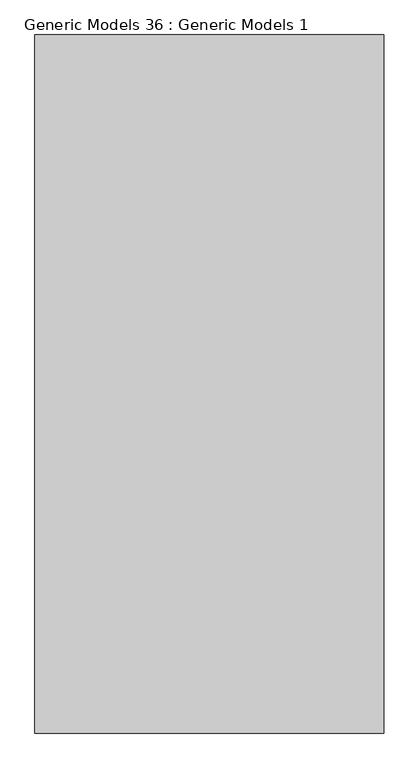
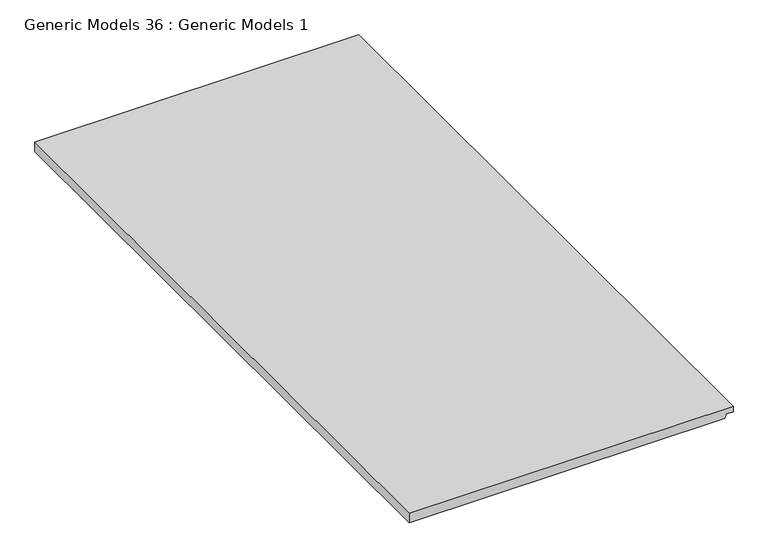
"""IFC4 building model written with IfcOpenShell, lengths in millimetres: proxy geometry, Generic Models 36 : Generic Models 1."""

from ifc_helpers import new_model, si_unit, frame, origin, place, context, project, spatial, polyline, outline, extrude, source, transform, mapped, element, save


def generic_models_36_generic_models_1_28f40251(model_context):
    return source(origin(), model_context, "Body", "SweptSolid", [
        extrude(outline(polyline([(2253.330428, 49662.5798593), (2253.330428, 49052.9798593), (2234.280428, 49052.9798593), (2234.280428, 49646.9908455), (2242.217928, 49649.8798593), (2242.217928, 49662.5798593), (2253.330428, 49662.5798593)])), frame((0.0, 0.0, 0.0), z_axis=(0.0, 1.0, 0.0), x_axis=(0.0, 0.0, 1.0)), (0.0, 0.0, 1.0), 1219.2),
    ])


if __name__ == "__main__":
    model = new_model("IFC4")
    model_context = context("Model", 3, world=origin())
    ifc_project = project(units=[si_unit("LENGTHUNIT", "METRE", prefix="MILLI")], contexts=[model_context])
    site = spatial("IfcSite", under=ifc_project)
    building = spatial("IfcBuilding", under=site)
    placement = place(None, origin())
    generic_models_36_generic_models_1_shape = generic_models_36_generic_models_1_28f40251(model_context)
    element("IfcBuildingElementProxy", 1, Name="Generic Models 36 : Generic Models 1", ObjectType="Generic Models 36 : Generic Models 1", at=placement, inside=building, context=model_context, shape_type="MappedRepresentation", body=[
        mapped(generic_models_36_generic_models_1_shape, transform((0.0, 0.0, 0.0), x_axis=(1.0, 0.0, 0.0), y_axis=(0.0, 1.0, 0.0), z_axis=(0.0, 0.0, 1.0))),
    ])
    save(model, "model.ifc")

# Revit data of these elements
# Element 1 (IfcBuildingElementProxy, "Generic Models 36 : Generic Models 1")
#   Materials on its faces: "CEILING AS SCHEDULED"
# Materials
#   "CEILING AS SCHEDULED": class "Generic", colour RGB 255 255 255, transparency 0, Cost = 0
